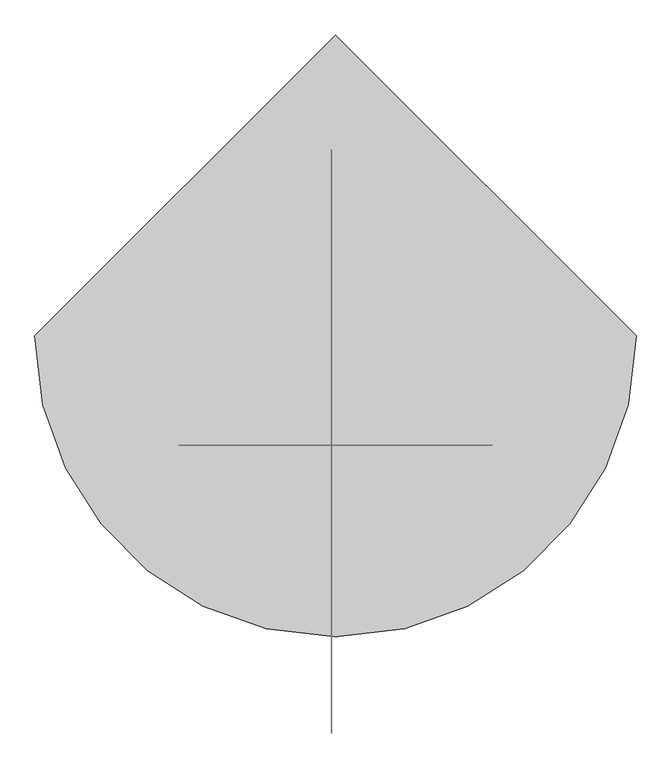
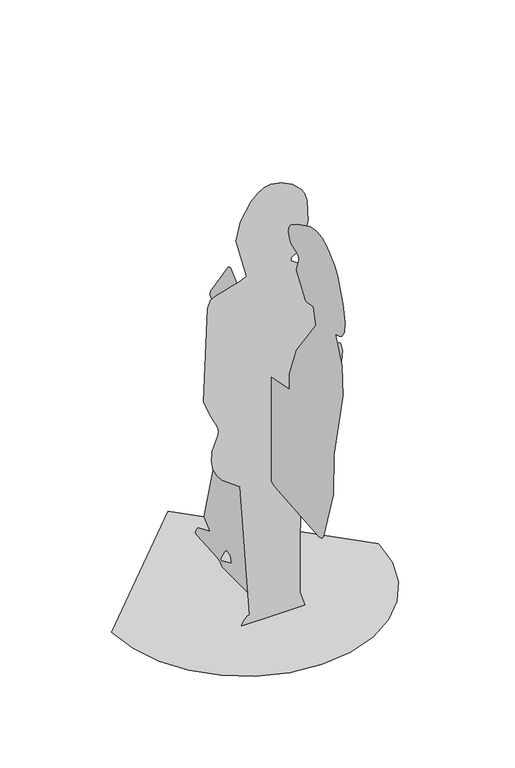
"""IFC4 building model written with IfcOpenShell, lengths in millimetres: proxy geometry, cynthia 25594 : cynthia 25594."""

import ifcopenshell
import ifcopenshell.guid

model = None  # the IFC model being written
_history = None  # IfcOwnerHistory: only IFC2X3 demands one
_inside = {}  # id of a spatial element -> (the spatial element, [elements in it])
_under = {}  # id of a project, library or spatial element -> (it, [spatial elements below it])
_declared = {}  # id of a project -> (the project, [libraries it declares])
_typed = {}  # id of a type object -> (the type object, [elements of that type])
_made_of = {}  # id of a material, layer set ... -> (it, [elements and type objects made of it])


def new_model(schema):
    """Start an empty IFC model of exactly this schema.

    Asked for "IFC4X3", IfcOpenShell would pick the latest addendum, in which some entities
    have other attributes; the version numbers below select the first issue.
    IFC2X3 requires an IfcOwnerHistory on every rooted entity: one is made here for all.
    """
    global model, _history
    if schema == "IFC4X3":
        model = ifcopenshell.file(schema_version=(4, 3, 0, 0))
    else:
        model = ifcopenshell.file(schema=schema)
    _inside.clear()
    _under.clear()
    _declared.clear()
    _typed.clear()
    _made_of.clear()
    _history = None
    if model.schema == "IFC2X3":
        org = make("IfcOrganization", Name="unknown")
        user = make(
            "IfcPersonAndOrganization",
            ThePerson=make("IfcPerson", FamilyName="unknown"),
            TheOrganization=org,
        )
        app = make(
            "IfcApplication",
            ApplicationDeveloper=org,
            Version="unknown",
            ApplicationFullName="unknown",
            ApplicationIdentifier="unknown",
        )
        _history = make(
            "IfcOwnerHistory",
            OwningUser=user,
            OwningApplication=app,
            ChangeAction="ADDED",
            CreationDate=0,
        )
    return model


def make(cls, **values):
    """One entity of the class cls with the attributes given. An attribute that is None is left unset."""
    return model.create_entity(
        cls, **{name: value for name, value in values.items() if value is not None}
    )


def rooted(cls, **values):
    """An entity with a GlobalId (a new one), such as an element, a storey or a relation."""
    return make(cls, GlobalId=ifcopenshell.guid.new(), OwnerHistory=_history, **values)


def si_unit(unit_type, name, prefix=None):
    """IfcSIUnit, for example si_unit("LENGTHUNIT", "METRE", prefix="MILLI")."""
    return make("IfcSIUnit", UnitType=unit_type, Prefix=prefix, Name=name)


def assignment(units):
    """IfcUnitAssignment: the units of a project."""
    return None if units is None else make("IfcUnitAssignment", Units=units)


def point(xyz):
    """IfcCartesianPoint."""
    return None if xyz is None else make("IfcCartesianPoint", Coordinates=xyz)


def direction(xyz):
    """IfcDirection."""
    return None if xyz is None else make("IfcDirection", DirectionRatios=xyz)


def frame(location, z_axis=None, x_axis=None):
    """IfcAxis2Placement3D, a coordinate frame: its origin and axes. An axis left out is left unset."""
    return make(
        "IfcAxis2Placement3D",
        Location=point(location),
        Axis=direction(z_axis),
        RefDirection=direction(x_axis),
    )


def origin():
    """The frame at (0, 0, 0) with its axes left unset."""
    return frame((0.0, 0.0, 0.0))


def place(relative_to, where):
    """IfcLocalPlacement: puts the frame where relative to a parent placement (None: the world)."""
    return make(
        "IfcLocalPlacement", PlacementRelTo=relative_to, RelativePlacement=where
    )


def context(
    kind, dimensions, precision=None, world=None, true_north=None, identifier=None
):
    """IfcGeometricRepresentationContext, for example the 3D "Model" context."""
    return make(
        "IfcGeometricRepresentationContext",
        ContextIdentifier=identifier,
        ContextType=kind,
        CoordinateSpaceDimension=dimensions,
        Precision=precision,
        WorldCoordinateSystem=world,
        TrueNorth=true_north,
    )


def project(units=None, contexts=None):
    """IfcProject with its units and contexts."""
    return rooted(
        "IfcProject",
        Name="project",
        RepresentationContexts=contexts,
        UnitsInContext=assignment(units),
    )


def spatial(cls, under=None, at=None, **own):
    """A site, building, storey or space (cls), placed at a placement, below another one or the project."""
    s = rooted(cls, ObjectPlacement=at, **own)
    if under is not None:
        _under.setdefault(under.id(), (under, []))[1].append(s)
    return s


def point_list(points):
    """IfcCartesianPointList2D or 3D."""
    cls = (
        "IfcCartesianPointList2D" if len(points[0]) == 2 else "IfcCartesianPointList3D"
    )
    return make(cls, CoordList=points)


def triangles(points, corners, closed=None, point_numbers=None):
    """IfcTriangulatedFaceSet: each triangle names its three corners, points numbered from 1."""
    return make(
        "IfcTriangulatedFaceSet",
        Coordinates=point_list(points),
        Closed=closed,
        CoordIndex=corners,
        PnIndex=point_numbers,
    )


def shape(context_of_items, identifier, shape_type, items):
    """IfcShapeRepresentation: the items that make up one representation, for example the "Body"."""
    return make(
        "IfcShapeRepresentation",
        ContextOfItems=context_of_items,
        RepresentationIdentifier=identifier,
        RepresentationType=shape_type,
        Items=items,
    )


def source(mapping_origin, context_of_items, identifier, shape_type, items):
    """IfcRepresentationMap: a shape defined once, which mapped items show again and again."""
    return make(
        "IfcRepresentationMap",
        MappingOrigin=mapping_origin,
        MappedRepresentation=shape(context_of_items, identifier, shape_type, items),
    )


def transform(
    local_origin,
    x_axis=None,
    y_axis=None,
    z_axis=None,
    scale=None,
    scale2=None,
    scale3=None,
    uniform=True,
):
    """IfcCartesianTransformationOperator3D, or its non-uniform kind. x_axis, y_axis, z_axis: its Axis1, 2, 3."""
    if uniform:
        return make(
            "IfcCartesianTransformationOperator3D",
            Axis1=direction(x_axis),
            Axis2=direction(y_axis),
            LocalOrigin=point(local_origin),
            Scale=scale,
            Axis3=direction(z_axis),
        )
    return make(
        "IfcCartesianTransformationOperator3DnonUniform",
        Axis1=direction(x_axis),
        Axis2=direction(y_axis),
        LocalOrigin=point(local_origin),
        Scale=scale,
        Axis3=direction(z_axis),
        Scale2=scale2,
        Scale3=scale3,
    )


def mapped(mapping_source, mapping_target):
    """IfcMappedItem: shows the shape of a source again, moved by a transform."""
    return make(
        "IfcMappedItem", MappingSource=mapping_source, MappingTarget=mapping_target
    )


def made_of(thing, what):
    """Note that an element or type object is made of a material, layer set ...; save() writes the relation."""
    if what is not None:
        _made_of.setdefault(what.id(), (what, []))[1].append(thing)
    return thing


def element(
    cls,
    number,
    at=None,
    inside=None,
    cuts=None,
    type_object=None,
    material=None,
    context=None,
    identifier="Body",
    shape_type=None,
    held_by="IfcProductDefinitionShape",
    body=None,
    shapes=None,
    **own,
):
    """One element of the class cls, such as IfcWall. Its Tag is "e" and its number.

    at: its placement. inside: the storey or other place that contains it. cuts: it is an
    opening in that element (IfcRelVoidsElement). A single representation is given by context,
    identifier, shape_type and body (its items); several are given by shapes. held_by: the class
    of the entity that holds the representations. save() writes the other relations.
    """
    e = rooted(cls, Tag="e%d" % number, ObjectPlacement=at, **own)
    if body is not None:
        shapes = [shape(context, identifier, shape_type, body)]
    if shapes is not None:
        e.Representation = make(held_by, Representations=shapes)
    if inside is not None:
        _inside.setdefault(inside.id(), (inside, []))[1].append(e)
    if cuts is not None:
        rooted(
            "IfcRelVoidsElement", RelatingBuildingElement=cuts, RelatedOpeningElement=e
        )
    if type_object is not None:
        _typed.setdefault(type_object.id(), (type_object, []))[1].append(e)
    return made_of(e, material)


def aggregate(whole, parts):
    """IfcRelAggregates: a whole, such as a stair, and the parts it consists of."""
    return rooted("IfcRelAggregates", RelatingObject=whole, RelatedObjects=parts)


def save(model, path):
    """Write the relations noted so far, then the file.

    IfcRelAggregates (storeys below a building ...), IfcRelContainedInSpatialStructure (elements
    in a storey), IfcRelDefinesByType, IfcRelAssociatesMaterial and IfcRelDeclares: one each for
    every whole, place, type object, material and project.
    """
    for whole, parts in _under.values():
        aggregate(whole, parts)
    for where, things in _inside.values():
        rooted(
            "IfcRelContainedInSpatialStructure",
            RelatedElements=things,
            RelatingStructure=where,
        )
    for kind, things in _typed.values():
        rooted("IfcRelDefinesByType", RelatedObjects=things, RelatingType=kind)
    for what, things in _made_of.values():
        rooted("IfcRelAssociatesMaterial", RelatedObjects=things, RelatingMaterial=what)
    for by, libraries in _declared.values():
        rooted("IfcRelDeclares", RelatingContext=by, RelatedDefinitions=libraries)
    model.write(path)


def entourage_c1b6233a(model_context):
    return source(origin(), model_context, "Body", "Tessellation", [
        triangles([(-437.3057565, 0.0, 2.93e-05), (-425.7448342, -100.2015691, 2.93e-05), (-392.8194094, -192.2206617, 2.93e-05), (-341.1658762, -273.4208834, 2.93e-05), (-273.4209015, -341.1659489, 2.93e-05), (-192.2206254, -392.819373, 2.93e-05), (-100.2015237, -425.7447616, 2.93e-05), (1.91e-05, -437.3057565, 2.93e-05), (100.2015782, -425.7448342, 2.93e-05), (192.220698, -392.8194094, 2.93e-05), (273.4209015, -341.1658762, 2.93e-05), (341.1660215, -273.4209015, 2.93e-05), (392.819373, -192.2206072, 2.93e-05), (425.7447616, -100.2014965, 2.93e-05), (437.3057565, 3.36e-05, 2.93e-05), (-5.73e-05, 437.3057928, 2.93e-05), (-5.5814555, 72.2468665, 69.496344), (-5.5814561, 67.0311374, 46.0256608), (-5.5814578, 124.4039163, 19.9471336), (-5.5814578, 129.6196227, 25.1628196), (-5.5814566, 107.6002182, 62.2269339), (-5.5814561, 95.7175496, 74.7120321), (-5.5814561, -28.6037069, 4.4e-06), (-5.5814549, -39.8908654, 35.5942482), (-5.5814549, -42.4985551, 37.2668205), (-5.5814544, -45.6385706, 39.1827964), (-5.5814544, -48.9915363, 41.1595652), (-5.5814544, -52.2381223, 43.0148345), (-5.5814544, -55.0589122, 44.56573), (-5.5814544, -57.134603, 45.6302408), (-5.5814544, -58.1458059, 46.0256654), (-5.5814555, -58.1458831, 5.3e-06), (-5.5814549, -108.953415, 6.8e-06), (-5.5814538, -116.5758059, 29.8220192), (-5.5814504, -109.3236867, 163.616957), (-5.5814407, -45.4571545, 488.7457126), (-5.5814407, -47.7144295, 510.223653), (-5.5814407, -52.9301177, 512.8314517), (-5.5814402, -176.6935208, 461.1352976), (-5.5814368, -431.0100288, 441.4516153), (-5.5814368, -446.7160832, 445.0272692), (-5.5814362, -456.1585665, 455.8251566), (-5.58143, -511.6809042, 636.0529638), (-5.581426, -514.5202658, 776.2247131), (-5.581418, -566.767113, 1012.4528086), (-5.5814152, -561.4616592, 1112.6378271), (-5.5814129, -522.3438071, 1198.6969637), (-5.5814124, -544.7658397, 1204.5966036), (-5.5814118, -561.2097124, 1214.9815075), (-5.5814112, -573.9143148, 1236.2570984), (-5.5814101, -577.4586843, 1272.8740494), (-5.5814084, -566.4219306, 1329.2823795), (-5.5814067, -535.3830548, 1409.9331253), (-5.5814061, -516.7871696, 1433.7636475), (-5.5814055, -472.5754423, 1474.3203289), (-5.5814055, -445.9831701, 1486.7813416), (-5.5814061, -415.7490054, 1491.187904), (-5.5814067, -381.3846059, 1485.4068615), (-5.5814084, -308.1102267, 1450.1702042), (-5.5814101, -271.6907564, 1426.3735462), (-5.5814101, -259.9822596, 1410.5514015), (-5.5814112, -256.5008769, 1391.3528641), (-5.5814118, -264.1662884, 1368.2074745), (-5.5814118, -270.5525991, 1361.5164585), (-5.5814118, -307.4893707, 1345.9730759), (-5.5814118, -313.689501, 1341.0963387), (-5.5814118, -316.3233155, 1334.3053288), (-5.5814124, -314.5104538, 1321.5896805), (-5.5814141, -303.2841223, 1289.971843), (-5.5814141, -303.9328654, 1281.3184467), (-5.5814146, -344.8551496, 1227.4567635), (-5.5814152, -350.2254976, 1216.9518814), (-5.5814152, -354.0100413, 1213.1371433), (-5.5814152, -360.9104559, 1211.8310457), (-5.5814141, -397.1668548, 1216.9518814), (-5.5814158, -412.8139375, 1162.1869829), (-5.581422, -300.7217424, 1007.464959), (-5.581426, -262.9221964, 903.7018885), (-5.5814271, -261.5584715, 849.2446747), (-5.58143, -151.2454011, 828.1021425), (-5.58143, -131.1657765, 828.3817766), (-5.5814283, -146.9133073, 873.4846922), (-5.5814283, -146.8128955, 875.3230974), (-5.5814283, -136.5283852, 880.5989382), (-5.581426, 66.2908483, 1062.7618017), (-5.581426, 72.9541816, 1068.1172161), (-5.581426, 85.3175848, 1063.7718418), (-5.5814322, 186.9119923, 916.7356859), (-5.5814322, 189.6002729, 904.0094278), (-5.5814339, 74.8547106, 802.3032085), (-5.5814345, 53.5231683, 768.5290346), (-5.5814345, 40.9526102, 757.9697227), (-5.5814345, 7.0502408, 750.1462177), (-5.5814362, -30.739564, 681.3427139), (-5.5814362, -32.0672787, 677.1262562), (-5.5814362, -2.7970168, 673.1418337), (-5.5814379, 74.8547106, 666.6947708), (-5.5814566, 223.5023279, 113.8298525), (-5.5814566, 192.3027424, 86.4272282), (-5.5814566, 189.6002729, 82.5355962), (-5.5814589, 257.4045281, 53.849234), (-5.5814589, 261.0572667, 50.6335418), (-5.5814595, 266.9932052, 41.9573409), (-5.58146, 270.4022813, 33.1798288), (-5.58146, 270.8965462, 29.8373162), (-5.58146, 270.443685, 27.7706614), (-5.58146, 262.21192, 24.6723948), (-5.5814583, 148.3989361, 17.7234776), (-5.5814583, 129.6196227, 12.1235582), (-5.5814583, 119.2279423, 0.0), (-103.2161017, -158.8625234, 3.138314), (-93.5649194, -158.8625234, 19.2429797), (-88.6211895, -158.8625234, 24.4594264), (-82.9717705, -158.8625234, 28.4095146), (-76.7113605, -158.8625234, 30.3784918), (-108.0056077, -158.8625597, 484.1449033), (-166.5178156, -158.8625597, 527.9969141), (-183.6322324, -158.8625597, 549.73316), (-196.1559229, -158.8625597, 575.232294), (-202.0512026, -158.8625597, 604.6165833), (-199.2805142, -158.8625597, 638.0082951), (-180.7337175, -158.8625597, 688.9249546), (-179.5104273, -158.8625597, 700.1737593), (-181.025542, -158.8625597, 711.0281839), (-186.0298695, -158.8625597, 724.8027792), (-192.7431225, -158.8625597, 739.7135696), (-208.5562016, -158.8625597, 771.7148867), (-227.9668628, -158.8625597, 820.5580536), (-215.5926544, -158.8625961, 1139.7188776), (-204.4961842, -158.8625961, 1164.7947453), (-195.70417, -158.8625961, 1170.2243557), (-178.399812, -158.8625961, 1176.5898829), (-156.0960135, -158.8625961, 1183.43634), (-132.3055416, -158.8625961, 1190.3076502), (-110.5412996, -158.8625961, 1196.7492628), (-94.3160908, -158.8625961, 1202.3053917), (-87.1427732, -158.8625961, 1206.520396), (-121.0448735, -158.8625961, 1339.5208534), (-105.9598114, -158.8626324, 1402.4766037), (-72.2006302, -158.8626324, 1459.3927517), (-51.1398881, -158.8626324, 1480.6086079), (-28.7965572, -158.8626324, 1494.3413452), (-6.2993123, -158.8626324, 1498.5999516), (28.3785912, -158.8626324, 1491.3003971), (62.9443683, -158.8626324, 1473.3394295), (92.2084342, -158.8626324, 1445.5309525), (103.2305721, -158.8626324, 1428.187825), (112.1216264, -158.8626324, 1400.9896305), (114.2135136, -158.8625961, 1329.2264236), (96.1614451, -158.8625961, 1258.9090588), (79.8725593, -158.8625961, 1233.5183121), (58.89705, -158.8625961, 1219.5597164), (58.89705, -158.8625961, 1209.1281584), (105.4402574, -158.8625961, 1177.1569994), (186.6818646, -158.8625961, 1146.5396095), (190.9101676, -158.8625961, 1130.2527403), (197.4604945, -158.8625961, 874.5613707), (217.1151996, -158.8625961, 870.6124111), (219.4354431, -158.8625961, 869.5265762), (221.3548754, -158.8625961, 866.986179), (227.9668991, -158.8625597, 839.7665468), (217.9761027, -158.8625597, 726.675412), (216.778683, -158.8625597, 725.5368914), (198.418848, -158.8625597, 721.3532078), (197.1132773, -158.8625597, 721.4595966), (188.2934486, -158.8625597, 736.0849394), (176.2504519, -158.8625597, 750.1460724), (172.5434834, -158.8625597, 744.3783285), (169.4576071, -158.8625597, 737.6237263), (166.7654749, -158.8625597, 730.2866741), (164.2397025, -158.8625597, 722.7717258), (161.6530689, -158.8625597, 715.4834352), (158.7781536, -158.8625597, 708.8262108), (155.3876083, -158.8625597, 703.2046062), (164.5987648, -158.8625597, 582.3864358), (159.7288041, -158.8625597, 557.9936296), (150.1719292, -158.8625597, 536.3020394), (143.452145, -158.8625597, 528.6085773), (105.433708, -158.8625597, 509.5447337), (96.8765541, -158.8625597, 503.2554374), (90.1912608, -158.8625597, 494.5763523), (88.7455914, -158.8625234, 49.4103652), (105.4365966, -158.8625234, 7.4e-05), (-104.3910027, -158.8625234, 7.4e-05)], [[15, 16, 1], [14, 15, 1], [14, 1, 2], [13, 14, 2], [13, 2, 3], [13, 3, 4], [12, 13, 4], [11, 12, 4], [11, 4, 5], [11, 5, 6], [11, 6, 7], [11, 7, 8], [11, 8, 9], [11, 9, 10], [23, 17, 18], [110, 23, 18], [110, 18, 19], [109, 110, 19], [17, 23, 24], [31, 32, 33], [31, 33, 34], [109, 19, 20], [108, 109, 20], [88, 89, 90], [82, 83, 84], [85, 86, 87], [105, 106, 107], [104, 105, 107], [103, 104, 107], [102, 103, 107], [101, 102, 107], [100, 101, 107], [100, 107, 108], [100, 108, 20], [100, 20, 21], [100, 21, 22], [87, 88, 90], [85, 87, 90], [84, 85, 90], [84, 90, 91], [84, 91, 92], [84, 92, 93], [82, 84, 93], [81, 82, 93], [81, 93, 94], [80, 81, 94], [80, 94, 95], [99, 100, 22], [17, 24, 25], [17, 25, 26], [31, 34, 35], [30, 31, 35], [17, 26, 27], [17, 27, 28], [17, 28, 29], [29, 30, 35], [17, 29, 35], [22, 17, 35], [99, 22, 35], [98, 99, 35], [97, 98, 35], [97, 35, 36], [97, 36, 37], [96, 97, 37], [96, 37, 38], [95, 96, 38], [80, 95, 38], [80, 38, 39], [79, 80, 39], [79, 39, 40], [79, 40, 41], [79, 41, 42], [79, 42, 43], [79, 43, 44], [78, 79, 44], [77, 78, 44], [77, 44, 45], [77, 45, 46], [76, 77, 46], [76, 46, 47], [75, 76, 47], [72, 73, 74], [71, 72, 74], [61, 62, 63], [60, 61, 63], [60, 63, 64], [59, 60, 64], [59, 64, 65], [59, 65, 66], [58, 59, 66], [57, 58, 66], [56, 57, 66], [55, 56, 66], [54, 55, 66], [54, 66, 67], [53, 54, 67], [52, 53, 67], [52, 67, 68], [51, 52, 68], [50, 51, 68], [49, 50, 68], [48, 49, 68], [47, 48, 68], [75, 47, 68], [74, 75, 68], [71, 74, 68], [70, 71, 68], [69, 70, 68], [183, 184, 111], [183, 111, 112], [183, 112, 113], [183, 113, 114], [183, 114, 115], [182, 183, 115], [181, 182, 115], [181, 115, 116], [154, 155, 156], [164, 165, 166], [180, 181, 116], [163, 164, 166], [162, 163, 166], [162, 166, 167], [161, 162, 167], [160, 161, 167], [159, 160, 167], [158, 159, 167], [157, 158, 167], [180, 116, 117], [180, 117, 118], [180, 118, 119], [180, 119, 120], [180, 120, 121], [180, 121, 122], [179, 180, 122], [179, 122, 123], [178, 179, 123], [177, 178, 123], [176, 177, 123], [175, 176, 123], [174, 175, 123], [174, 123, 124], [174, 124, 125], [173, 174, 125], [172, 173, 125], [171, 172, 125], [170, 171, 125], [169, 170, 125], [169, 125, 126], [168, 169, 126], [168, 126, 127], [167, 168, 127], [157, 167, 127], [157, 127, 128], [156, 157, 128], [154, 156, 128], [153, 154, 128], [153, 128, 129], [153, 129, 130], [153, 130, 131], [153, 131, 132], [153, 132, 133], [153, 133, 134], [153, 134, 135], [153, 135, 136], [153, 136, 137], [152, 153, 137], [151, 152, 137], [150, 151, 137], [149, 150, 137], [149, 137, 138], [149, 138, 139], [148, 149, 139], [147, 148, 139], [146, 147, 139], [146, 139, 140], [145, 146, 140], [145, 140, 141], [144, 145, 141], [144, 141, 142], [144, 142, 143]], closed=False),
    ])


if __name__ == "__main__":
    model = new_model("IFC4")
    model_context = context("Model", 3, world=origin())
    ifc_project = project(units=[si_unit("LENGTHUNIT", "METRE", prefix="MILLI")], contexts=[model_context])
    site = spatial("IfcSite", under=ifc_project)
    building = spatial("IfcBuilding", under=site)
    placement = place(None, origin())
    entourage_shape = entourage_c1b6233a(model_context)
    element("IfcBuildingElementProxy", 1, Name="cynthia 25594 : cynthia 25594", ObjectType="cynthia 25594 : cynthia 25594", at=placement, inside=building, context=model_context, shape_type="MappedRepresentation", body=[
        mapped(entourage_shape, transform((0.0, 0.0, 0.0), x_axis=(1.0, 0.0, 0.0), y_axis=(0.0, 1.0, 0.0), z_axis=(0.0, 0.0, 1.0))),
    ])
    save(model, "model.ifc")

# Revit data of these elements
# Type "cynthia 25594 : cynthia 25594"
#   built-in parameter 1005195 = "RPC-8-FXA2-QQQ0-UGV2-6"
#   Height = 0
